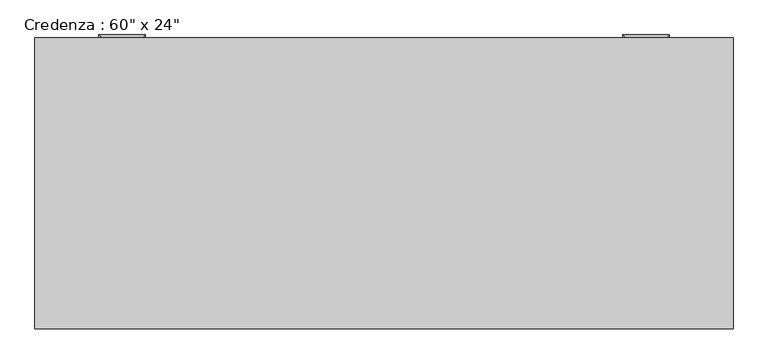
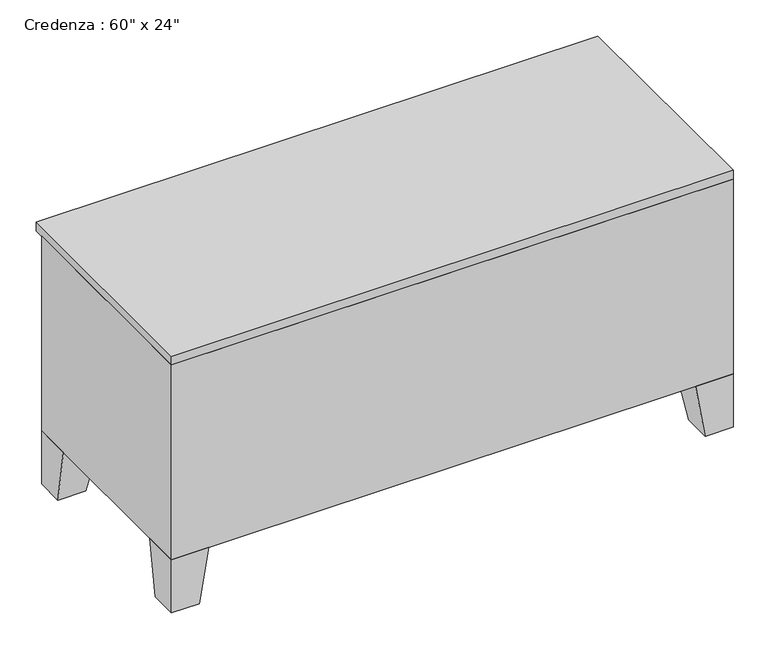
"""IFC4 building model written with IfcOpenShell, lengths in millimetres: furniture geometry."""

from ifc_helpers import new_model, si_unit, frame, origin, place, context, project, spatial, polyline, outline, extrude, faceted_brep, source, transform, mapped, element, save


def furniture_a9e97cbc(model_context):
    return source(origin(), model_context, "Body", "SolidModel", [
        extrude(outline(polyline([(455.5023176, 267.2714583), (455.5023176, 254.5714583), (46.8442623, 254.5714583), (46.8442623, 267.2714583), (455.5023176, 267.2714583)])), frame((0.0, 0.0, 171.45), z_axis=(0.0, 0.0, 1.0), x_axis=(1.0, 0.0, 0.0)), (0.0, 0.0, 1.0), 520.7),
        extrude(outline(polyline([(73.6254475, 279.9714583), (73.6254475, 267.2714583), (-302.4057377, 267.2714583), (-302.4057377, 279.9714583), (73.6254475, 279.9714583)])), frame((0.0, 0.0, 171.45), z_axis=(0.0, 0.0, 1.0), x_axis=(1.0, 0.0, 0.0)), (0.0, 0.0, 1.0), 520.7),
        faceted_brep([(719.9442623, -309.3803279, 152.4), (821.5442623, -309.3803279, 152.4), (821.5442623, -207.7803279, 152.4), (719.9442623, -207.7803279, 152.4), (745.3442623, -309.3803279, 0.0), (745.3442623, -233.1803279, 0.0), (821.5442623, -233.1803279, 0.0), (821.5442623, -309.3803279, 0.0)], [[[0, 1, 2, 3]], [[4, 5, 6, 7]], [[4, 0, 3, 5]], [[5, 3, 2, 6]], [[6, 2, 1, 7]], [[7, 1, 0, 4]]]),
        extrude(outline(polyline([(802.4942623, 306.5696721), (802.4942623, 300.2196721), (440.5442623, 300.2196721), (440.5442623, 306.5696721), (802.4942623, 306.5696721)])), frame((0.0, 0.0, 584.2), z_axis=(0.0, 0.0, 1.0), x_axis=(1.0, 0.0, 0.0)), (0.0, 0.0, 1.0), 107.95),
        extrude(outline(polyline([(802.4942623, 306.5696721), (802.4942623, 300.2196721), (440.5442623, 300.2196721), (440.5442623, 306.5696721), (802.4942623, 306.5696721)])), frame((0.0, 0.0, 171.45), z_axis=(0.0, 0.0, 1.0), x_axis=(1.0, 0.0, 0.0)), (0.0, 0.0, 1.0), 393.7),
        extrude(outline(polyline([(-321.4557377, 306.5696721), (-321.4557377, 300.2196721), (-683.4057377, 300.2196721), (-683.4057377, 306.5696721), (-321.4557377, 306.5696721)])), frame((0.0, 0.0, 584.2), z_axis=(0.0, 0.0, 1.0), x_axis=(1.0, 0.0, 0.0)), (0.0, 0.0, 1.0), 107.95),
        extrude(outline(polyline([(-321.4557377, 306.5696721), (-321.4557377, 300.2196721), (-683.4057377, 300.2196721), (-683.4057377, 306.5696721), (-321.4557377, 306.5696721)])), frame((0.0, 0.0, 171.45), z_axis=(0.0, 0.0, 1.0), x_axis=(1.0, 0.0, 0.0)), (0.0, 0.0, 1.0), 393.7),
        faceted_brep([(-600.8557377, 300.2196721, 152.4), (-702.4557377, 300.2196721, 152.4), (-702.4557377, 198.6196721, 152.4), (-600.8557377, 198.6196721, 152.4), (-626.2557377, 300.2196721, 0.0), (-626.2557377, 224.0196721, 0.0), (-702.4557377, 224.0196721, 0.0), (-702.4557377, 300.2196721, 0.0)], [[[0, 1, 2, 3]], [[4, 5, 6, 7]], [[4, 0, 3, 5]], [[5, 3, 2, 6]], [[6, 2, 1, 7]], [[7, 1, 0, 4]]]),
        faceted_brep([(-600.8557377, -309.3803279, 152.4), (-600.8557377, -207.7803279, 152.4), (-702.4557377, -207.7803279, 152.4), (-702.4557377, -309.3803279, 152.4), (-626.2557377, -309.3803279, 0.0), (-702.4557377, -309.3803279, 0.0), (-702.4557377, -233.1803279, 0.0), (-626.2557377, -233.1803279, 0.0)], [[[0, 1, 2, 3]], [[4, 5, 6, 7]], [[4, 0, 3, 5]], [[5, 3, 2, 6]], [[6, 2, 1, 7]], [[7, 1, 0, 4]]]),
        faceted_brep([(719.9442623, 300.2196721, 152.4), (719.9442623, 198.6196721, 152.4), (821.5442623, 198.6196721, 152.4), (821.5442623, 300.2196721, 152.4), (745.3442623, 300.2196721, 0.0), (821.5442623, 300.2196721, 0.0), (821.5442623, 224.0196721, 0.0), (745.3442623, 224.0196721, 0.0)], [[[0, 1, 2, 3]], [[4, 5, 6, 7]], [[4, 0, 3, 5]], [[5, 3, 2, 6]], [[6, 2, 1, 7]], [[7, 1, 0, 4]]]),
        faceted_brep([(821.5442623, -309.3803279, 711.2), (821.5442623, 300.2196721, 711.2), (-702.4557377, 300.2196721, 711.2), (-702.4557377, -309.3803279, 711.2), (821.5442623, -309.3803279, 152.4), (-702.4557377, -309.3803279, 152.4), (-702.4557377, 300.2196721, 152.4), (821.5442623, 300.2196721, 152.4), (-302.4057377, 300.2196721, 692.15), (-302.4057377, 300.2196721, 171.45), (421.4942623, 300.2196721, 171.45), (421.4942623, 300.2196721, 692.15), (421.4942623, -290.3303279, 692.15), (421.4942623, -290.3303279, 171.45), (-302.4057377, -290.3303279, 171.45), (-302.4057377, -290.3303279, 692.15)], [[[0, 1, 2, 3]], [[4, 5, 6, 7]], [[3, 5, 4, 0]], [[2, 6, 5, 3]], [[1, 7, 6, 2], [8, 9, 10, 11]], [[0, 4, 7, 1]], [[12, 13, 14, 15]], [[15, 8, 11, 12]], [[14, 9, 8, 15]], [[13, 10, 9, 14]], [[12, 11, 10, 13]]]),
        extrude(outline(polyline([(821.5442623, -309.3803279), (-702.4557377, -309.3803279), (-702.4557377, 325.6196721), (821.5442623, 325.6196721), (821.5442623, -309.3803279)])), frame((0.0, 0.0, 711.2), z_axis=(0.0, 0.0, 1.0), x_axis=(1.0, 0.0, 0.0)), (0.0, 0.0, 1.0), 25.4),
        faceted_brep([(-556.4057377, 306.5696721, 527.05), (-562.7557377, 306.5696721, 527.05), (-562.7557377, 306.5696721, 514.35), (-556.4057377, 306.5696721, 514.35), (-556.4057377, 325.6196721, 514.35), (-556.4057377, 325.6196721, 527.05), (-562.7557377, 331.9696721, 514.35), (-562.7557377, 331.9696721, 527.05), (-467.5057377, 325.6196721, 514.35), (-467.5057377, 325.6196721, 527.05), (-461.1557377, 331.9696721, 514.35), (-461.1557377, 331.9696721, 527.05), (-467.5057377, 306.5696721, 527.05), (-467.5057377, 306.5696721, 514.35), (-461.1557377, 306.5696721, 514.35), (-461.1557377, 306.5696721, 527.05)], [[[0, 1, 2, 3]], [[3, 4, 5, 0]], [[2, 6, 4, 3]], [[1, 7, 6, 2]], [[0, 5, 7, 1]], [[4, 8, 9, 5]], [[6, 10, 8, 4]], [[7, 11, 10, 6]], [[5, 9, 11, 7]], [[12, 13, 14, 15]], [[8, 13, 12, 9]], [[10, 14, 13, 8]], [[11, 15, 14, 10]], [[9, 12, 15, 11]]]),
        faceted_brep([(-556.4057377, 306.5696721, 654.05), (-562.7557377, 306.5696721, 654.05), (-562.7557377, 306.5696721, 641.35), (-556.4057377, 306.5696721, 641.35), (-556.4057377, 325.6196721, 641.35), (-556.4057377, 325.6196721, 654.05), (-562.7557377, 331.9696721, 641.35), (-562.7557377, 331.9696721, 654.05), (-467.5057377, 325.6196721, 641.35), (-467.5057377, 325.6196721, 654.05), (-461.1557377, 331.9696721, 641.35), (-461.1557377, 331.9696721, 654.05), (-467.5057377, 306.5696721, 654.05), (-467.5057377, 306.5696721, 641.35), (-461.1557377, 306.5696721, 641.35), (-461.1557377, 306.5696721, 654.05)], [[[0, 1, 2, 3]], [[3, 4, 5, 0]], [[2, 6, 4, 3]], [[1, 7, 6, 2]], [[0, 5, 7, 1]], [[4, 8, 9, 5]], [[6, 10, 8, 4]], [[7, 11, 10, 6]], [[5, 9, 11, 7]], [[12, 13, 14, 15]], [[8, 13, 12, 9]], [[10, 14, 13, 8]], [[11, 15, 14, 10]], [[9, 12, 15, 11]]]),
        faceted_brep([(586.5942623, 306.5696721, 654.1373112), (580.2442623, 306.5696721, 654.1373112), (580.2442623, 306.5696721, 641.4373112), (586.5942623, 306.5696721, 641.4373112), (586.5942623, 325.6196721, 641.4373112), (586.5942623, 325.6196721, 654.1373112), (580.2442623, 331.9696721, 641.4373112), (580.2442623, 331.9696721, 654.1373112), (675.4942623, 325.6196721, 641.4373112), (675.4942623, 325.6196721, 654.1373112), (681.8442623, 331.9696721, 641.4373112), (681.8442623, 331.9696721, 654.1373112), (675.4942623, 306.5696721, 654.1373112), (675.4942623, 306.5696721, 641.4373112), (681.8442623, 306.5696721, 641.4373112), (681.8442623, 306.5696721, 654.1373112)], [[[0, 1, 2, 3]], [[3, 4, 5, 0]], [[2, 6, 4, 3]], [[1, 7, 6, 2]], [[0, 5, 7, 1]], [[4, 8, 9, 5]], [[6, 10, 8, 4]], [[7, 11, 10, 6]], [[5, 9, 11, 7]], [[12, 13, 14, 15]], [[8, 13, 12, 9]], [[10, 14, 13, 8]], [[11, 15, 14, 10]], [[9, 12, 15, 11]]]),
        faceted_brep([(586.5942623, 306.5696721, 527.05), (580.2442623, 306.5696721, 527.05), (580.2442623, 306.5696721, 514.35), (586.5942623, 306.5696721, 514.35), (586.5942623, 325.6196721, 514.35), (586.5942623, 325.6196721, 527.05), (580.2442623, 331.9696721, 514.35), (580.2442623, 331.9696721, 527.05), (675.4942623, 325.6196721, 514.35), (675.4942623, 325.6196721, 527.05), (681.8442623, 331.9696721, 514.35), (681.8442623, 331.9696721, 527.05), (675.4942623, 306.5696721, 527.05), (675.4942623, 306.5696721, 514.35), (681.8442623, 306.5696721, 514.35), (681.8442623, 306.5696721, 527.05)], [[[0, 1, 2, 3]], [[3, 4, 5, 0]], [[2, 6, 4, 3]], [[1, 7, 6, 2]], [[0, 5, 7, 1]], [[4, 8, 9, 5]], [[6, 10, 8, 4]], [[7, 11, 10, 6]], [[5, 9, 11, 7]], [[12, 13, 14, 15]], [[8, 13, 12, 9]], [[10, 14, 13, 8]], [[11, 15, 14, 10]], [[9, 12, 15, 11]]]),
    ])


if __name__ == "__main__":
    model = new_model("IFC4")
    model_context = context("Model", 3, world=origin())
    ifc_project = project(units=[si_unit("LENGTHUNIT", "METRE", prefix="MILLI")], contexts=[model_context])
    site = spatial("IfcSite", under=ifc_project)
    building = spatial("IfcBuilding", under=site)
    placement = place(None, origin())
    furniture_shape = furniture_a9e97cbc(model_context)
    element("IfcFurniture", 1, ObjectType="Credenza : 60\" x 24\"", at=placement, inside=building, context=model_context, shape_type="MappedRepresentation", body=[
        mapped(furniture_shape, transform((0.0, 0.0, 0.0), x_axis=(1.0, 0.0, 0.0), y_axis=(0.0, 1.0, 0.0), z_axis=(0.0, 0.0, 1.0))),
    ])
    save(model, "model.ifc")

# Revit data of these elements
# Type "Credenza : 60\" x 24\""
#   Assembly Code = "E2020200"
#   Depth = 2' - 0"
#   Height = 2' - 5"
#   Width = 5' - 0"
#   Body Material = Laminate, Ivory, Matte
#   Handles/Legs Material = Steel, Chrome Plated
#   Top Material = Cherry
#   Default Elevation = 0
# Element 1 (IfcFurniture, "Credenza : 60\" x 24\"")
#   Materials on its faces: "Steel, Chrome Plated", "Laminate, Ivory, Matte", "Cherry"
# Materials
#   "Laminate, Ivory, Matte": class "Plastic", colour RGB 247 247 239, transparency 0, Description = "Plastic Laminate - Ivory, Matte", Cost = 0
#   "Steel, Chrome Plated": class "Metal", colour RGB 17 17 17, transparency 0, Description = "Chromiuim plated steel", Cost = 0
#   "Cherry": class "Wood", colour RGB 226 177 128, transparency 0, Description = "Prunus Serotina", Cost = 0
